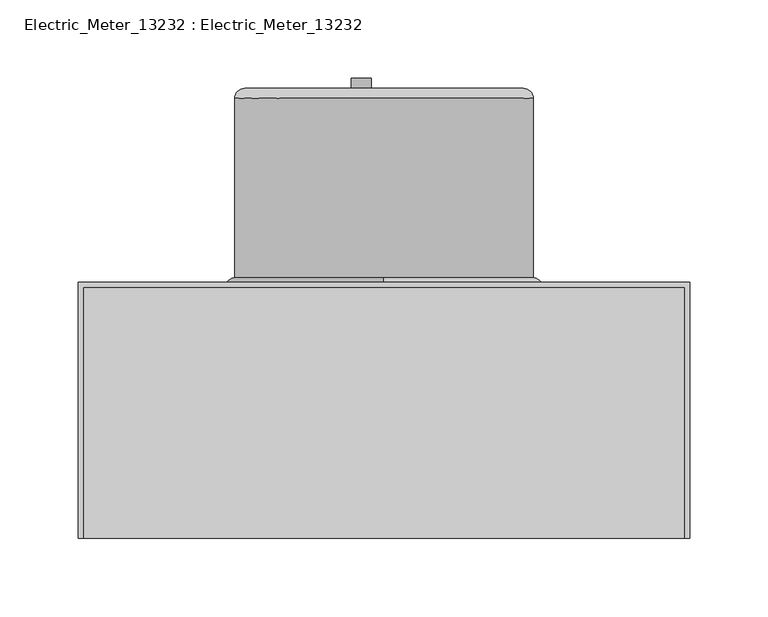
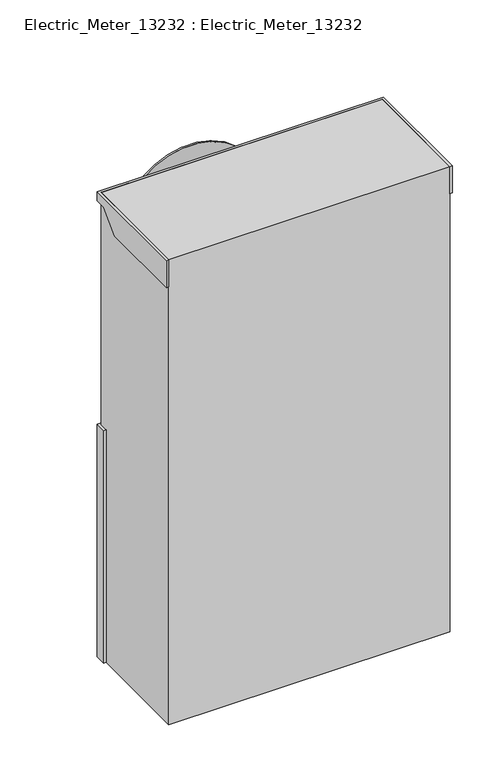
"""IFC4 building model written with IfcOpenShell, lengths in millimetres: proxy geometry, Electric_Meter_13232 : Electric_Meter_13232."""

from ifc_helpers import new_model, si_unit, point, frame, frame_2d, origin, place, context, project, spatial, polyline, circle_curve, ellipse_curve, trimmed, segment, composite_curve, outline, extrude, faceted_brep, source, transform, mapped, element, save
from ifc_brep_helpers import plane_surface, cylinder_surface, revolved_surface, advanced_brep


def electric_meter_13232_electric_meter_13232_95067e7f(model_context):
    return source(origin(), model_context, "Body", "SolidModel", [
        extrude(outline(composite_curve([segment(trimmed(circle_curve(frame_2d((1721.9414062, 0.0)), 82.55), [point((1721.9414062, 82.55))], [point((1721.9414062, -82.55))], False, "CARTESIAN"), True, "CONTINUOUS"), segment(trimmed(circle_curve(frame_2d((1721.9414062, 0.0)), 82.55), [point((1721.9414062, -82.55))], [point((1721.9414062, 82.55))], False, "CARTESIAN"), True, "CONTINUOUS")], self_intersect=False)), frame((0.0, 313.4320312, 0.0), z_axis=(0.0, 1.0, 0.0), x_axis=(0.0, 0.0, 1.0)), (0.0, 0.0, 1.0), 113.443562),
        advanced_brep(
        [(95.25, 313.4320312, 1721.9414062), (-95.25, 313.4320312, 1721.9414062), (93.6625, 313.4320312, 1721.9414062), (-93.6625, 313.4320312, 1721.9414062), (-95.25, 434.0820312, 1721.9414062), (95.25, 434.0820313, 1721.9414062), (-93.6625, 434.0820312, 1721.9414062), (93.6625, 434.0820313, 1721.9414062), (88.9, 438.8445313, 1721.9414062), (-88.9, 438.8445312, 1721.9414062), (88.9, 440.4320313, 1721.9414062), (-88.9, 440.4320312, 1721.9414062), (-8.1033428, 440.4320312, 1671.3092763), (-20.8033428, 440.4320312, 1671.3092763), (-17.0667397, 440.4320312, 1665.5219922), (-17.0667397, 440.4320312, 1652.2592763), (-11.8399458, 440.4320312, 1652.2592763), (-11.8399458, 440.4320312, 1665.5219922), (-20.8033428, 446.7820312, 1671.3092763), (-8.1033428, 446.7820312, 1671.3092763), (-11.8399458, 446.7820312, 1665.5219922), (-11.8399458, 446.7820312, 1654.3418459), (-17.0667397, 446.7820312, 1654.3418459), (-17.0667397, 446.7820312, 1665.5219922), (-17.0667397, 444.6994616, 1652.2592763), (-17.0667397, 443.6070312, 1660.5510914), (-17.0667397, 443.6070312, 1656.6674611), (-11.8399458, 444.6994616, 1652.2592763), (-11.8399458, 443.6070312, 1660.5510914), (-11.8399458, 443.6070312, 1656.6674611)],
        [
            (0, 1, circle_curve(frame((0.0, 313.4320312, 1721.9414062), z_axis=(0.0, -1.0, 0.0), x_axis=(-1.0, 0.0, 0.0)), 95.25)),
            (1, 0, circle_curve(frame((0.0, 313.4320312, 1721.9414062), z_axis=(0.0, -1.0, 0.0), x_axis=(-1.0, 0.0, 0.0)), 95.25)),
            (2, 3, circle_curve(frame((0.0, 313.4320312, 1721.9414062), z_axis=(0.0, 1.0, 0.0), x_axis=(-1.0, 0.0, 0.0)), 93.6625)),
            (3, 2, circle_curve(frame((0.0, 313.4320312, 1721.9414062), z_axis=(0.0, 1.0, 0.0), x_axis=(-1.0, 0.0, 0.0)), 93.6625)),
            (1, 4),
            (4, 5, circle_curve(frame((0.0, 434.0820313, 1721.9414062), z_axis=(0.0, -1.0, 0.0), x_axis=(-1.0, 0.0, 0.0)), 95.25)),
            (5, 0),
            (5, 4, circle_curve(frame((0.0, 434.0820313, 1721.9414062), z_axis=(0.0, -1.0, 0.0), x_axis=(-1.0, 0.0, 0.0)), 95.25)),
            (3, 6),
            (6, 7, circle_curve(frame((0.0, 434.0820313, 1721.9414062), z_axis=(0.0, 1.0, 0.0), x_axis=(-1.0, 0.0, 0.0)), 93.6625)),
            (7, 2),
            (7, 6, circle_curve(frame((0.0, 434.0820313, 1721.9414062), z_axis=(0.0, 1.0, 0.0), x_axis=(-1.0, 0.0, 0.0)), 93.6625)),
            (8, 7, circle_curve(frame((88.9, 434.0820313, 1721.9414062), z_axis=(0.0, 0.0, -1.0), x_axis=(-1.0, 0.0, 0.0)), 4.7625)),
            (6, 9, circle_curve(frame((-88.9, 434.0820312, 1721.9414062), z_axis=(0.0, 0.0, -1.0), x_axis=(1.0, 2.118024383194854e-12, 0.0)), 4.7625)),
            (9, 8, circle_curve(frame((0.0, 438.8445312, 1721.9414062), z_axis=(-1.059012191597427e-12, 1.0, 0.0), x_axis=(1.0, 1.059012191597427e-12, 0.0)), 88.9)),
            (8, 9, circle_curve(frame((0.0, 438.8445312, 1721.9414062), z_axis=(-1.059012191597427e-12, 1.0, 0.0), x_axis=(1.0, 1.059012191597427e-12, 0.0)), 88.9)),
            (5, 10, circle_curve(frame((88.9, 434.0820313, 1721.9414062), z_axis=(0.0, 0.0, 1.0), x_axis=(-1.0, 0.0, 0.0)), 6.35)),
            (10, 11, circle_curve(frame((0.0, 440.4320312, 1721.9414062), z_axis=(1.059012191597427e-12, -1.0, 0.0), x_axis=(1.0, 1.059012191597427e-12, 0.0)), 88.9)),
            (11, 4, circle_curve(frame((-88.9, 434.0820312, 1721.9414062), z_axis=(0.0, 0.0, 1.0), x_axis=(1.0, 2.118024383194854e-12, 0.0)), 6.35)),
            (11, 10, circle_curve(frame((0.0, 440.4320312, 1721.9414062), z_axis=(1.059012191597427e-12, -1.0, 0.0), x_axis=(1.0, 1.059012191597427e-12, 0.0)), 88.9)),
            (12, 13, circle_curve(frame((-14.4533428, 440.4320312, 1671.3092763), z_axis=(0.0, -1.0, 0.0), x_axis=(-1.0, 0.0, 0.0)), 6.35)),
            (13, 14, circle_curve(frame((-14.4533428, 440.4320312, 1671.3092763), z_axis=(0.0, -1.0, 0.0), x_axis=(-1.0, 0.0, 0.0)), 6.35)),
            (14, 15),
            (15, 16),
            (16, 17),
            (17, 12, circle_curve(frame((-14.4533428, 440.4320312, 1671.3092763), z_axis=(0.0, -1.0, 0.0), x_axis=(-1.0, 0.0, 0.0)), 6.35)),
            (18, 19, circle_curve(frame((-14.4533428, 446.7820312, 1671.3092763), z_axis=(0.0, 1.0, 0.0), x_axis=(-1.0, 0.0, 0.0)), 6.35)),
            (19, 20, circle_curve(frame((-14.4533428, 446.7820312, 1671.3092763), z_axis=(0.0, 1.0, 0.0), x_axis=(-1.0, 0.0, 0.0)), 6.35)),
            (20, 21),
            (21, 22),
            (22, 23),
            (23, 18, circle_curve(frame((-14.4533428, 446.7820312, 1671.3092763), z_axis=(0.0, 1.0, 0.0), x_axis=(-1.0, 0.0, 0.0)), 6.35)),
            (19, 12),
            (17, 20),
            (13, 18),
            (23, 14),
            (22, 24, circle_curve(frame((-17.0667397, 444.6994616, 1654.3418459), z_axis=(-1.0, 0.0, 0.0), x_axis=(0.0, 0.0, -1.0)), 2.0825696)),
            (24, 15),
            (25, 26, circle_curve(frame((-17.0667397, 443.6070312, 1658.6092763), z_axis=(1.0, 0.0, 0.0), x_axis=(0.0, 0.0, -1.0)), 1.9418151)),
            (26, 25, circle_curve(frame((-17.0667397, 443.6070312, 1658.6092763), z_axis=(1.0, 0.0, 0.0), x_axis=(0.0, 0.0, -1.0)), 1.9418151)),
            (16, 27),
            (27, 21, circle_curve(frame((-11.8399458, 444.6994616, 1654.3418459), z_axis=(1.0, 0.0, 0.0), x_axis=(0.0, 0.0, -1.0)), 2.0825696)),
            (28, 29, circle_curve(frame((-11.8399458, 443.6070312, 1658.6092763), z_axis=(-1.0, 0.0, 0.0), x_axis=(0.0, 0.0, -1.0)), 1.9418151)),
            (29, 28, circle_curve(frame((-11.8399458, 443.6070312, 1658.6092763), z_axis=(-1.0, 0.0, 0.0), x_axis=(0.0, 0.0, -1.0)), 1.9418151)),
            (27, 24),
            (25, 28),
            (29, 26),
        ],
        [
            plane_surface(frame((-95.25, 313.4320312, 1721.9414062), z_axis=(0.0, -1.0, 0.0), x_axis=(0.0, 0.0, -1.0))),
            cylinder_surface(frame((0.0, 313.4320312, 1721.9414062), z_axis=(0.0, 1.0, 0.0), x_axis=(-1.0, 0.0, 0.0)), 95.25),
            revolved_surface(polyline([(-93.6625, 313.4320312, 1721.9414062), (-93.6625, 434.0820313, 1721.9414062)]), (0.0, 313.4320312, 1721.9414062), (0.0, -1.0, 0.0)),
            revolved_surface(trimmed(ellipse_curve(frame((88.9, 434.0820313, 1721.9414062), z_axis=(0.0, 0.0, 1.0), x_axis=(-1.0, 0.0, 0.0)), 4.7625, 4.7625), [point((93.6625, 434.0820313, 1721.9414062))], [point((88.9, 438.8445313, 1721.9414062))], True, "CARTESIAN"), (0.0, 434.0820313, 1721.9414062), (1.059012191597427e-12, -1.0, 0.0)),
            revolved_surface(trimmed(ellipse_curve(frame((88.9, 434.0820313, 1721.9414062), z_axis=(0.0, 0.0, -1.0), x_axis=(-1.0, 0.0, 0.0)), 6.35, 6.35), [point((88.9, 440.4320313, 1721.9414062))], [point((95.25, 434.0820313, 1721.9414062))], True, "CARTESIAN"), (0.0, 434.0820313, 1721.9414062), (1.059012191597427e-12, -1.0, 0.0)),
            plane_surface(frame((88.9, 440.4320312, 1721.9414062), z_axis=(0.0, 1.0, 0.0), x_axis=(0.0, 0.0, -1.0))),
            plane_surface(frame((88.9, 438.8445312, 1721.9414062), z_axis=(0.0, -1.0, 0.0), x_axis=(0.0, 0.0, 1.0))),
            plane_surface(frame((-20.8033428, 446.7820312, 1671.3092763), z_axis=(0.0, 1.0, 0.0), x_axis=(0.0, 0.0, 1.0))),
            cylinder_surface(frame((-14.4533428, 440.4320312, 1671.3092763), z_axis=(0.0, 1.0, 0.0), x_axis=(-1.0, 0.0, 0.0)), 6.35),
            plane_surface(frame((-17.0667397, 446.7820312, 1666.8343807), z_axis=(-1.0, 0.0, 0.0), x_axis=(0.0, 1.0, 0.0))),
            plane_surface(frame((-11.8399458, 446.7820312, 1666.8343807), z_axis=(1.0, 0.0, 0.0), x_axis=(0.0, -1.0, 0.0))),
            cylinder_surface(frame((-11.8399458, 444.6994616, 1654.3418459), z_axis=(-1.0, 0.0, 0.0), x_axis=(0.0, 0.0, -1.0)), 2.0825696),
            plane_surface(frame((-17.0667397, 444.6994616, 1652.2592763), z_axis=(0.0, 0.0, -1.0), x_axis=(1.0, 0.0, 0.0))),
            revolved_surface(polyline([(-11.8399458, 443.6070312, 1656.6674612), (-17.0667397, 443.6070312, 1656.6674612)]), (0.0, 443.6070312, 1658.6092763), (1.0, 0.0, 0.0)),
        ],
        [
            (0, [[1, 2], [3, 4]]),
            (1, [[-2, 5, 6, 7]]),
            (1, [[-1, -7, 8, -5]]),
            (2, [[-4, 9, 10, 11]]),
            (2, [[-3, -11, 12, -9]]),
            (3, [[13, -10, 14, 15]]),
            (3, [[-13, 16, -14, -12]]),
            (4, [[17, 18, 19, -8]]),
            (4, [[-17, -6, -19, 20]]),
            (5, [[-18, -20], [21, 22, 23, 24, 25, 26]]),
            (6, [[-15, -16]]),
            (7, [[27, 28, 29, 30, 31, 32]]),
            (8, [[33, -26, 34, -28]]),
            (8, [[35, -32, 36, -22]]),
            (8, [[-27, -35, -21, -33]]),
            (9, [[37, 38, -23, -36, -31], [39, 40]]),
            (10, [[41, 42, -29, -34, -25], [43, 44]]),
            (11, [[-37, -30, -42, 45]]),
            (12, [[-38, -45, -41, -24]]),
            (13, [[-39, 46, -44, 47]]),
            (13, [[-40, -47, -43, -46]]),
        ],
    ),
        advanced_brep(
        [(0.0, 313.4320312, 1626.6914062), (0.0, 313.4320312, 1817.1914062), (0.0, 319.7820312, 1817.1914062), (0.0, 319.7820312, 1626.6914062), (0.0, 313.4320312, 1620.3414062), (0.0, 313.4320312, 1823.5414062)],
        [
            (0, 1, circle_curve(frame((0.0, 313.4320312, 1721.9414062), z_axis=(0.0, -1.0, 0.0), x_axis=(0.0, 0.0, 1.0)), 95.25)),
            (1, 2),
            (2, 3, circle_curve(frame((0.0, 319.7820312, 1721.9414062), z_axis=(0.0, 1.0, 0.0), x_axis=(0.0, 0.0, 1.0)), 95.25)),
            (3, 0),
            (1, 0, circle_curve(frame((0.0, 313.4320312, 1721.9414062), z_axis=(0.0, -1.0, 0.0), x_axis=(0.0, 0.0, 1.0)), 95.25)),
            (3, 2, circle_curve(frame((0.0, 319.7820312, 1721.9414062), z_axis=(0.0, 1.0, 0.0), x_axis=(0.0, 0.0, 1.0)), 95.25)),
            (4, 5, circle_curve(frame((0.0, 313.4320312, 1721.9414062), z_axis=(0.0, -1.0, 0.0), x_axis=(0.0, 0.0, 1.0)), 101.6)),
            (5, 1),
            (0, 4),
            (5, 4, circle_curve(frame((0.0, 313.4320312, 1721.9414062), z_axis=(0.0, -1.0, 0.0), x_axis=(0.0, 0.0, 1.0)), 101.6)),
            (2, 5, circle_curve(frame((0.0, 313.4320312, 1817.1914062), z_axis=(1.0, 0.0, 0.0), x_axis=(0.0, 0.0, -1.0)), 6.35)),
            (4, 3, circle_curve(frame((0.0, 313.4320312, 1626.6914062), z_axis=(1.0, 0.0, 0.0), x_axis=(0.0, 0.0, 1.0)), 6.35)),
        ],
        [
            revolved_surface(polyline([(0.0, 319.7820312, 1817.1914062), (0.0, 313.4320312, 1817.1914062)]), (0.0, 313.4320312, 1721.9414062), (0.0, 1.0, 0.0)),
            plane_surface(frame((0.0, 313.4320312, 1721.9414062), z_axis=(0.0, -1.0, 0.0), x_axis=(0.0, 0.0, 1.0))),
            revolved_surface(trimmed(ellipse_curve(frame((0.0, 313.4320312, 1817.1914062), z_axis=(-1.0, 0.0, 0.0), x_axis=(0.0, 0.0, -1.0)), 6.35, 6.35), [point((0.0, 313.4320312, 1823.5414062))], [point((0.0, 319.7820312, 1817.1914062))], True, "CARTESIAN"), (0.0, 313.4320312, 1721.9414062), (0.0, 1.0, 0.0)),
        ],
        [
            (0, [[1, 2, 3, 4]]),
            (0, [[5, -4, 6, -2]]),
            (1, [[7, 8, -1, 9]]),
            (1, [[10, -9, -5, -8]]),
            (2, [[-3, 11, -7, 12]]),
            (2, [[-6, -12, -10, -11]]),
        ],
    ),
        extrude(outline(polyline([(-195.0640625, 301.4871664), (-195.0640625, 316.6070312), (195.0640625, 316.6070312), (195.0640625, 301.4871664), (191.8890625, 301.4871664), (191.8890625, 313.4320312), (-191.8890625, 313.4320312), (-191.8890625, 301.4871664), (-195.0640625, 301.4871664)])), frame((0.0, 0.0, 1219.2), z_axis=(0.0, 0.0, 1.0), x_axis=(1.0, 0.0, 0.0)), (0.0, 0.0, 1.0), 335.1609375),
        faceted_brep([(191.8890625, 301.4871664, 1876.821875), (191.8890625, 275.3320313, 1850.6667399), (191.8890625, 153.19375, 1850.6667399), (191.8890625, 153.19375, 1889.521875), (191.8890625, 313.4320312, 1889.521875), (191.8890625, 313.4320312, 1876.821875), (195.0640625, 301.4871664, 1876.821875), (195.0640625, 316.6070313, 1876.821875), (195.0640625, 316.6070313, 1889.521875), (195.0640625, 153.19375, 1889.521875), (195.0640625, 153.19375, 1850.6667399), (195.0640625, 275.3320313, 1850.6667399), (-191.8890625, 313.4320313, 1876.821875), (-191.8890625, 301.4871664, 1876.821875), (-195.0640625, 301.4871664, 1876.821875), (-195.0640625, 316.6070312, 1876.821875), (-195.0640625, 316.6070312, 1889.521875), (-195.0640625, 153.19375, 1889.521875), (-191.8890625, 153.19375, 1889.521875), (-191.8890625, 313.4320313, 1889.521875), (-191.8890625, 153.19375, 1850.6667399), (-191.8890625, 275.3320312, 1850.6667399), (-195.0640625, 275.3320312, 1850.6667399), (-195.0640625, 153.19375, 1850.6667399)], [[[0, 1, 2, 3, 4, 5]], [[6, 7, 8, 9, 10, 11]], [[7, 6, 0, 5, 12, 13, 14, 15]], [[9, 8, 16, 17, 18, 19, 4, 3]], [[3, 2, 10, 9]], [[2, 1, 11, 10]], [[1, 0, 6, 11]], [[16, 8, 7, 15]], [[4, 19, 12, 5]], [[18, 20, 21, 13, 12, 19]], [[14, 22, 23, 17, 16, 15]], [[20, 18, 17, 23]], [[21, 20, 23, 22]], [[13, 21, 22, 14]]]),
        extrude(outline(polyline([(322.9570312, 1308.1), (329.3070312, 1301.75), (329.3070312, 1289.05), (322.9570312, 1282.7), (316.6070312, 1282.7), (316.6070312, 1308.1), (322.9570312, 1308.1)]), holes=[composite_curve([segment(trimmed(circle_curve(frame_2d((322.9570312, 1295.4)), 3.1560846), [point((319.8009466, 1295.4))], [point((326.1131159, 1295.4))], True, "CARTESIAN"), True, "CONTINUOUS"), segment(trimmed(circle_curve(frame_2d((322.9570312, 1295.4)), 3.1560846), [point((326.1131159, 1295.4))], [point((319.8009466, 1295.4))], True, "CARTESIAN"), True, "CONTINUOUS")], self_intersect=False)]), frame((-1.5875, 0.0, 0.0), z_axis=(1.0, 0.0, 0.0), x_axis=(0.0, 1.0, 0.0)), (0.0, 0.0, 1.0), 3.175),
        extrude(outline(polyline([(191.8890625, 153.19375), (-191.8890625, 153.19375), (-191.8890625, 313.4320312), (191.8890625, 313.4320312), (191.8890625, 153.19375)])), frame((0.0, 0.0, 1219.2), z_axis=(0.0, 0.0, 1.0), x_axis=(1.0, 0.0, 0.0)), (0.0, 0.0, 1.0), 670.321875),
    ])


if __name__ == "__main__":
    model = new_model("IFC4")
    model_context = context("Model", 3, world=origin())
    ifc_project = project(units=[si_unit("LENGTHUNIT", "METRE", prefix="MILLI")], contexts=[model_context])
    site = spatial("IfcSite", under=ifc_project)
    building = spatial("IfcBuilding", under=site)
    placement = place(None, origin())
    electric_meter_13232_electric_meter_13232_shape = electric_meter_13232_electric_meter_13232_95067e7f(model_context)
    element("IfcBuildingElementProxy", 1, Name="Electric_Meter_13232 : Electric_Meter_13232", ObjectType="Electric_Meter_13232 : Electric_Meter_13232", at=placement, inside=building, context=model_context, shape_type="MappedRepresentation", body=[
        mapped(electric_meter_13232_electric_meter_13232_shape, transform((0.0, 0.0, 0.0), x_axis=(1.0, 0.0, 0.0), y_axis=(0.0, 1.0, 0.0), z_axis=(0.0, 0.0, 1.0))),
    ])
    save(model, "model.ifc")

# Revit data of these elements
# Type "Electric_Meter_13232 : Electric_Meter_13232"
#   Overall Width = 1' - 3 7/64"
#   Overall Height = 2' - 2 25/64"
#   Overall Depth = 0' - 6 79/256"
#   Offset From Wall [instance default] = 0' - 6"
#   Height AFF [instance default] = 4' - 0"
#   Box Material = ELECTRICAL METERS
# Element 1 (IfcBuildingElementProxy, "Electric_Meter_13232 : Electric_Meter_13232")
#   Offset From Wall = 0' - 0"
#   Materials on its faces: "ELECTRICAL METERS", "06 64 00_PLASTIC_TRANSPARENT_CLEAR_POLISHED", "05 00 00_CHROME_POLISHED", "26 27 26_RECEPTACLE FACE PLATE_WHITE"
# Materials
#   "ELECTRICAL METERS": class "Generic", colour RGB 120 120 120, transparency 0, Cost = 0
#   "06 64 00_PLASTIC_TRANSPARENT_CLEAR_POLISHED": class "Unassigned", colour RGB 192 192 192, transparency 0, Comments = "Rendering appearance not upgraded ", Description = "Concrete"
#   "05 00 00_CHROME_POLISHED": class "Miscellaneous", colour RGB 244 244 244, transparency 0
#   "26 27 26_RECEPTACLE FACE PLATE_WHITE": class "Plastic", colour RGB 249 249 249, transparency 0
